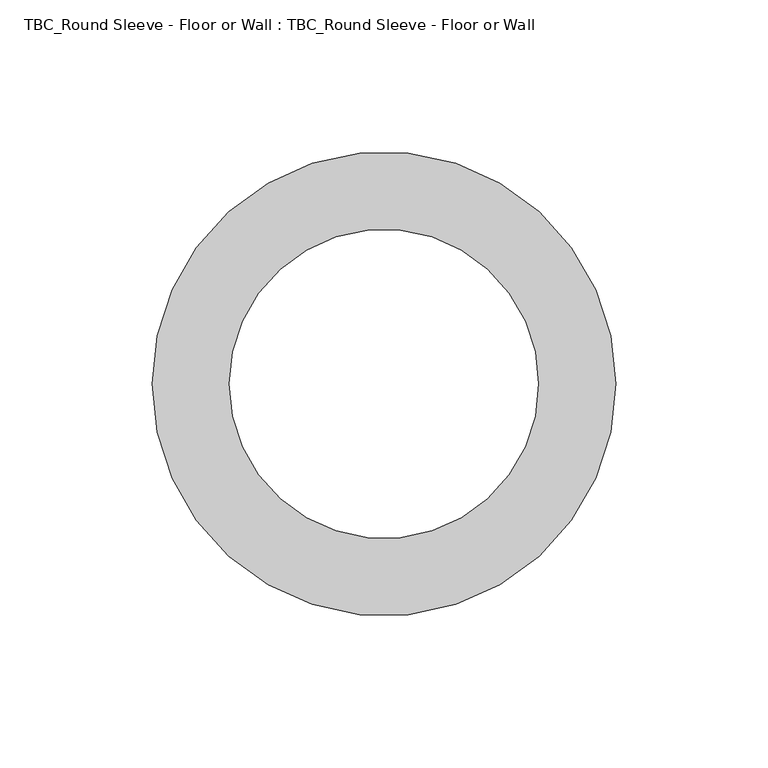
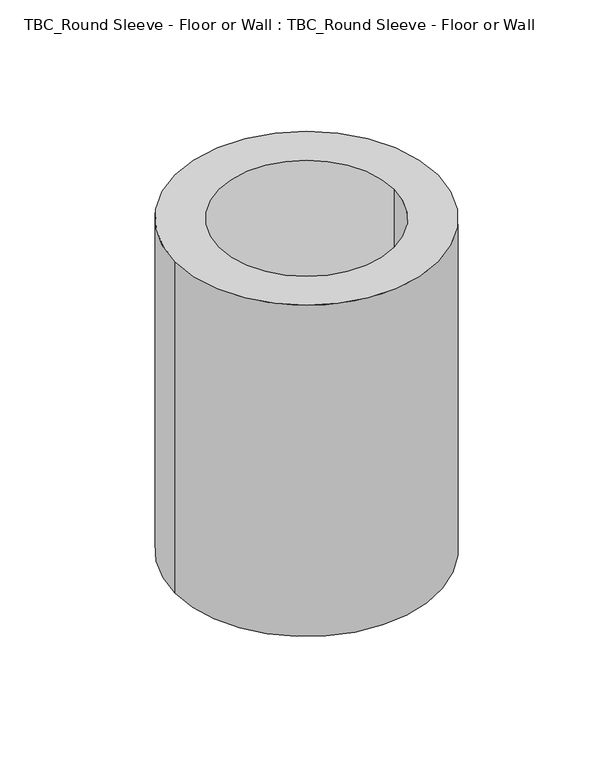
"""IFC4 building model written with IfcOpenShell, lengths in millimetres: proxy geometry, TBC_Round Sleeve - Floor or Wall : TBC_Round Sleeve - Floor or Wall."""

from ifc_helpers import new_model, si_unit, point, frame, origin, origin_2d, place, context, project, spatial, circle_curve, trimmed, segment, composite_curve, outline, extrude, source, transform, mapped, element, save


def tbc_round_sleeve_floor_or_wall_tbc_round_sleeve_floor_or_f81fbc2f(model_context):
    return source(origin(), model_context, "Body", "SweptSolid", [
        extrude(outline(composite_curve([segment(trimmed(circle_curve(origin_2d(), 76.2), [point((-76.2, 0.0))], [point((76.2, 0.0))], False, "CARTESIAN"), True, "CONTINUOUS"), segment(trimmed(circle_curve(origin_2d(), 76.2), [point((76.2, 0.0))], [point((-76.2, 0.0))], False, "CARTESIAN"), True, "CONTINUOUS")], self_intersect=False), holes=[composite_curve([segment(trimmed(circle_curve(origin_2d(), 50.8), [point((-50.8, 0.0))], [point((50.8, 0.0))], True, "CARTESIAN"), True, "CONTINUOUS"), segment(trimmed(circle_curve(origin_2d(), 50.8), [point((50.8, 0.0))], [point((-50.8, 0.0))], True, "CARTESIAN"), True, "CONTINUOUS")], self_intersect=False)]), frame((0.0, 0.0, -203.2), z_axis=(0.0, 0.0, 1.0), x_axis=(1.0, 0.0, 0.0)), (0.0, 0.0, 1.0), 203.2),
    ])


if __name__ == "__main__":
    model = new_model("IFC4")
    model_context = context("Model", 3, world=origin())
    ifc_project = project(units=[si_unit("LENGTHUNIT", "METRE", prefix="MILLI")], contexts=[model_context])
    site = spatial("IfcSite", under=ifc_project)
    building = spatial("IfcBuilding", under=site)
    placement = place(None, origin())
    tbc_round_sleeve_floor_or_wall_tbc_round_sleeve_floor_or_shape = tbc_round_sleeve_floor_or_wall_tbc_round_sleeve_floor_or_f81fbc2f(model_context)
    element("IfcBuildingElementProxy", 1, Name="TBC_Round Sleeve - Floor or Wall : TBC_Round Sleeve - Floor or Wall", ObjectType="TBC_Round Sleeve - Floor or Wall : TBC_Round Sleeve - Floor or Wall", at=placement, inside=building, context=model_context, shape_type="MappedRepresentation", body=[
        mapped(tbc_round_sleeve_floor_or_wall_tbc_round_sleeve_floor_or_shape, transform((0.0, 0.0, 0.0), x_axis=(1.0, 0.0, 0.0), y_axis=(0.0, 1.0, 0.0), z_axis=(0.0, 0.0, 1.0))),
    ])
    save(model, "model.ifc")

# Revit data of these elements
# Type "TBC_Round Sleeve - Floor or Wall : TBC_Round Sleeve - Floor or Wall"
#   Tag Dimension [instance default] = ""
#   MEP Type [instance default] = ""
#   MEP Element [instance default] = ""
#   MEP Category [instance default] = ""
#   Host Element Type [instance default] = ""
#   Host Element Id [instance default] = ""
#   Host Element Category [instance default] = ""
#   Control Line Y [instance default] = ""
#   Control Line X [instance default] = ""
#   Sleeve Radius [instance default] = 1' - 0"
#   Sleeve Edge [instance default] = 1' - 2"
#   Sleeve Depth [instance default] = 3' - 0"
#   Distance Y [instance default] = 0' - 0"
#   Distance X [instance default] = 0' - 0"
#   Default Elevation = 0
# Element 1 (IfcBuildingElementProxy, "TBC_Round Sleeve - Floor or Wall : TBC_Round Sleeve - Floor or Wall")
#   Tag Dimension = "6\""
#   MEP Type = "PLG-S"
#   MEP Element = "1012458"
#   MEP Category = "Pipe"
#   Host Element Type = "8\" Plank"
#   Host Element Id = "529506"
#   Host Element Category = "Floors"
#   Sleeve Radius = 0' - 4"
#   Sleeve Edge = 0' - 6"
#   Sleeve Depth = 0' - 8"
